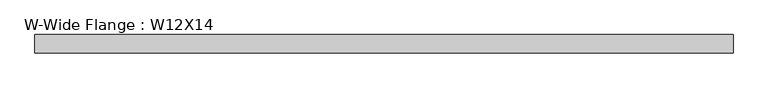
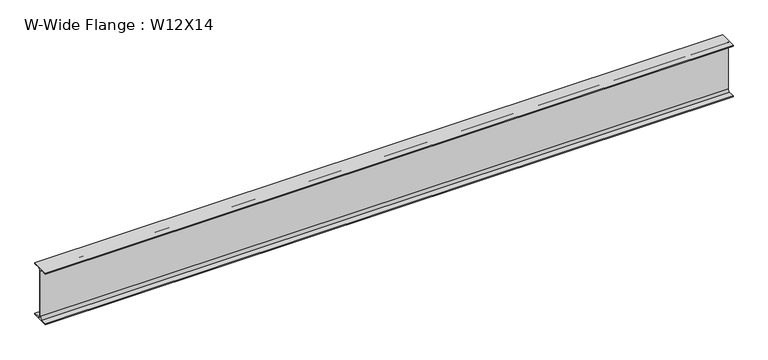
"""IFC4 building model written with IfcOpenShell, lengths in millimetres: beam geometry, W-Wide Flange : W12X14."""

import ifcopenshell
import ifcopenshell.guid

model = None  # the IFC model being written
_history = None  # IfcOwnerHistory: only IFC2X3 demands one
_inside = {}  # id of a spatial element -> (the spatial element, [elements in it])
_under = {}  # id of a project, library or spatial element -> (it, [spatial elements below it])
_declared = {}  # id of a project -> (the project, [libraries it declares])
_typed = {}  # id of a type object -> (the type object, [elements of that type])
_made_of = {}  # id of a material, layer set ... -> (it, [elements and type objects made of it])


def new_model(schema):
    """Start an empty IFC model of exactly this schema.

    Asked for "IFC4X3", IfcOpenShell would pick the latest addendum, in which some entities
    have other attributes; the version numbers below select the first issue.
    IFC2X3 requires an IfcOwnerHistory on every rooted entity: one is made here for all.
    """
    global model, _history
    if schema == "IFC4X3":
        model = ifcopenshell.file(schema_version=(4, 3, 0, 0))
    else:
        model = ifcopenshell.file(schema=schema)
    _inside.clear()
    _under.clear()
    _declared.clear()
    _typed.clear()
    _made_of.clear()
    _history = None
    if model.schema == "IFC2X3":
        org = make("IfcOrganization", Name="unknown")
        user = make(
            "IfcPersonAndOrganization",
            ThePerson=make("IfcPerson", FamilyName="unknown"),
            TheOrganization=org,
        )
        app = make(
            "IfcApplication",
            ApplicationDeveloper=org,
            Version="unknown",
            ApplicationFullName="unknown",
            ApplicationIdentifier="unknown",
        )
        _history = make(
            "IfcOwnerHistory",
            OwningUser=user,
            OwningApplication=app,
            ChangeAction="ADDED",
            CreationDate=0,
        )
    return model


def make(cls, **values):
    """One entity of the class cls with the attributes given. An attribute that is None is left unset."""
    return model.create_entity(
        cls, **{name: value for name, value in values.items() if value is not None}
    )


def rooted(cls, **values):
    """An entity with a GlobalId (a new one), such as an element, a storey or a relation."""
    return make(cls, GlobalId=ifcopenshell.guid.new(), OwnerHistory=_history, **values)


def si_unit(unit_type, name, prefix=None):
    """IfcSIUnit, for example si_unit("LENGTHUNIT", "METRE", prefix="MILLI")."""
    return make("IfcSIUnit", UnitType=unit_type, Prefix=prefix, Name=name)


def assignment(units):
    """IfcUnitAssignment: the units of a project."""
    return None if units is None else make("IfcUnitAssignment", Units=units)


def point(xyz):
    """IfcCartesianPoint."""
    return None if xyz is None else make("IfcCartesianPoint", Coordinates=xyz)


def direction(xyz):
    """IfcDirection."""
    return None if xyz is None else make("IfcDirection", DirectionRatios=xyz)


def frame(location, z_axis=None, x_axis=None):
    """IfcAxis2Placement3D, a coordinate frame: its origin and axes. An axis left out is left unset."""
    return make(
        "IfcAxis2Placement3D",
        Location=point(location),
        Axis=direction(z_axis),
        RefDirection=direction(x_axis),
    )


def frame_2d(location, x_axis=None):
    """IfcAxis2Placement2D, a coordinate frame in the plane: its origin and x axis."""
    return make(
        "IfcAxis2Placement2D", Location=point(location), RefDirection=direction(x_axis)
    )


def origin():
    """The frame at (0, 0, 0) with its axes left unset."""
    return frame((0.0, 0.0, 0.0))


def place(relative_to, where):
    """IfcLocalPlacement: puts the frame where relative to a parent placement (None: the world)."""
    return make(
        "IfcLocalPlacement", PlacementRelTo=relative_to, RelativePlacement=where
    )


def context(
    kind, dimensions, precision=None, world=None, true_north=None, identifier=None
):
    """IfcGeometricRepresentationContext, for example the 3D "Model" context."""
    return make(
        "IfcGeometricRepresentationContext",
        ContextIdentifier=identifier,
        ContextType=kind,
        CoordinateSpaceDimension=dimensions,
        Precision=precision,
        WorldCoordinateSystem=world,
        TrueNorth=true_north,
    )


def project(units=None, contexts=None):
    """IfcProject with its units and contexts."""
    return rooted(
        "IfcProject",
        Name="project",
        RepresentationContexts=contexts,
        UnitsInContext=assignment(units),
    )


def spatial(cls, under=None, at=None, **own):
    """A site, building, storey or space (cls), placed at a placement, below another one or the project."""
    s = rooted(cls, ObjectPlacement=at, **own)
    if under is not None:
        _under.setdefault(under.id(), (under, []))[1].append(s)
    return s


def polyline(points):
    """IfcPolyline through the points."""
    return make("IfcPolyline", Points=[point(p) for p in points])


def circle_curve(where, radius):
    """IfcCircle in the frame where."""
    return make("IfcCircle", Position=where, Radius=radius)


def trimmed(basis, trim1, trim2, sense, master):
    """IfcTrimmedCurve: the piece of a basis curve between two trims."""
    return make(
        "IfcTrimmedCurve",
        BasisCurve=basis,
        Trim1=trim1,
        Trim2=trim2,
        SenseAgreement=sense,
        MasterRepresentation=master,
    )


def segment(curve, same_sense, transition):
    """IfcCompositeCurveSegment."""
    return make(
        "IfcCompositeCurveSegment",
        Transition=transition,
        SameSense=same_sense,
        ParentCurve=curve,
    )


def composite_curve(segments, self_intersect=None):
    """IfcCompositeCurve: segments joined end to end."""
    return make("IfcCompositeCurve", Segments=segments, SelfIntersect=self_intersect)


def outline(outer, holes=None, kind="AREA"):
    """IfcArbitraryClosedProfileDef: a profile drawn as a closed curve; with holes, ...WithVoids."""
    if holes is None:
        return make("IfcArbitraryClosedProfileDef", ProfileType=kind, OuterCurve=outer)
    return make(
        "IfcArbitraryProfileDefWithVoids",
        ProfileType=kind,
        OuterCurve=outer,
        InnerCurves=holes,
    )


def extrude(swept, where, along, depth):
    """IfcExtrudedAreaSolid: the profile swept, set in the frame where, extruded along a direction by depth."""
    return make(
        "IfcExtrudedAreaSolid",
        SweptArea=swept,
        Position=where,
        ExtrudedDirection=direction(along),
        Depth=depth,
    )


def shape(context_of_items, identifier, shape_type, items):
    """IfcShapeRepresentation: the items that make up one representation, for example the "Body"."""
    return make(
        "IfcShapeRepresentation",
        ContextOfItems=context_of_items,
        RepresentationIdentifier=identifier,
        RepresentationType=shape_type,
        Items=items,
    )


def source(mapping_origin, context_of_items, identifier, shape_type, items):
    """IfcRepresentationMap: a shape defined once, which mapped items show again and again."""
    return make(
        "IfcRepresentationMap",
        MappingOrigin=mapping_origin,
        MappedRepresentation=shape(context_of_items, identifier, shape_type, items),
    )


def transform(
    local_origin,
    x_axis=None,
    y_axis=None,
    z_axis=None,
    scale=None,
    scale2=None,
    scale3=None,
    uniform=True,
):
    """IfcCartesianTransformationOperator3D, or its non-uniform kind. x_axis, y_axis, z_axis: its Axis1, 2, 3."""
    if uniform:
        return make(
            "IfcCartesianTransformationOperator3D",
            Axis1=direction(x_axis),
            Axis2=direction(y_axis),
            LocalOrigin=point(local_origin),
            Scale=scale,
            Axis3=direction(z_axis),
        )
    return make(
        "IfcCartesianTransformationOperator3DnonUniform",
        Axis1=direction(x_axis),
        Axis2=direction(y_axis),
        LocalOrigin=point(local_origin),
        Scale=scale,
        Axis3=direction(z_axis),
        Scale2=scale2,
        Scale3=scale3,
    )


def mapped(mapping_source, mapping_target):
    """IfcMappedItem: shows the shape of a source again, moved by a transform."""
    return make(
        "IfcMappedItem", MappingSource=mapping_source, MappingTarget=mapping_target
    )


def made_of(thing, what):
    """Note that an element or type object is made of a material, layer set ...; save() writes the relation."""
    if what is not None:
        _made_of.setdefault(what.id(), (what, []))[1].append(thing)
    return thing


def element(
    cls,
    number,
    at=None,
    inside=None,
    cuts=None,
    type_object=None,
    material=None,
    context=None,
    identifier="Body",
    shape_type=None,
    held_by="IfcProductDefinitionShape",
    body=None,
    shapes=None,
    **own,
):
    """One element of the class cls, such as IfcWall. Its Tag is "e" and its number.

    at: its placement. inside: the storey or other place that contains it. cuts: it is an
    opening in that element (IfcRelVoidsElement). A single representation is given by context,
    identifier, shape_type and body (its items); several are given by shapes. held_by: the class
    of the entity that holds the representations. save() writes the other relations.
    """
    e = rooted(cls, Tag="e%d" % number, ObjectPlacement=at, **own)
    if body is not None:
        shapes = [shape(context, identifier, shape_type, body)]
    if shapes is not None:
        e.Representation = make(held_by, Representations=shapes)
    if inside is not None:
        _inside.setdefault(inside.id(), (inside, []))[1].append(e)
    if cuts is not None:
        rooted(
            "IfcRelVoidsElement", RelatingBuildingElement=cuts, RelatedOpeningElement=e
        )
    if type_object is not None:
        _typed.setdefault(type_object.id(), (type_object, []))[1].append(e)
    return made_of(e, material)


def aggregate(whole, parts):
    """IfcRelAggregates: a whole, such as a stair, and the parts it consists of."""
    return rooted("IfcRelAggregates", RelatingObject=whole, RelatedObjects=parts)


def save(model, path):
    """Write the relations noted so far, then the file.

    IfcRelAggregates (storeys below a building ...), IfcRelContainedInSpatialStructure (elements
    in a storey), IfcRelDefinesByType, IfcRelAssociatesMaterial and IfcRelDeclares: one each for
    every whole, place, type object, material and project.
    """
    for whole, parts in _under.values():
        aggregate(whole, parts)
    for where, things in _inside.values():
        rooted(
            "IfcRelContainedInSpatialStructure",
            RelatedElements=things,
            RelatingStructure=where,
        )
    for kind, things in _typed.values():
        rooted("IfcRelDefinesByType", RelatedObjects=things, RelatingType=kind)
    for what, things in _made_of.values():
        rooted("IfcRelAssociatesMaterial", RelatedObjects=things, RelatingMaterial=what)
    for by, libraries in _declared.values():
        rooted("IfcRelDeclares", RelatingContext=by, RelatedDefinitions=libraries)
    model.write(path)


def w_wide_flange_w12x14_02e3ecd4(model_context):
    return source(origin(), model_context, "Body", "SweptSolid", [
        extrude(outline(composite_curve([segment(polyline([(50.419, -145.415), (50.419, -151.13), (-50.419, -151.13), (-50.419, -145.415), (-15.875, -145.415)]), True, "CONTINUOUS"), segment(trimmed(circle_curve(frame_2d((-15.875, -132.08)), 13.335), [point((-15.875, -145.415))], [point((-2.54, -132.08))], True, "CARTESIAN"), True, "CONTINUOUS"), segment(polyline([(-2.54, -132.08), (-2.54, 132.08)]), True, "CONTINUOUS"), segment(trimmed(circle_curve(frame_2d((-15.875, 132.08)), 13.335), [point((-2.54, 132.08))], [point((-15.875, 145.415))], True, "CARTESIAN"), True, "CONTINUOUS"), segment(polyline([(-15.875, 145.415), (-50.419, 145.415), (-50.419, 151.13), (50.419, 151.13), (50.419, 145.415), (15.875, 145.415)]), True, "CONTINUOUS"), segment(trimmed(circle_curve(frame_2d((15.875, 132.08)), 13.335), [point((15.875, 145.415))], [point((2.54, 132.08))], True, "CARTESIAN"), True, "CONTINUOUS"), segment(polyline([(2.54, 132.08), (2.54, -132.08)]), True, "CONTINUOUS"), segment(trimmed(circle_curve(frame_2d((15.875, -132.08)), 13.335), [point((2.54, -132.08))], [point((15.875, -145.415))], True, "CARTESIAN"), True, "CONTINUOUS"), segment(polyline([(15.875, -145.415), (50.419, -145.415)]), True, "CONTINUOUS")], self_intersect=False)), frame((-1905.0, 0.0, 0.0), z_axis=(1.0, 0.0, 0.0), x_axis=(0.0, 1.0, 0.0)), (0.0, 0.0, 1.0), 3810.0),
    ])


if __name__ == "__main__":
    model = new_model("IFC4")
    model_context = context("Model", 3, world=origin())
    ifc_project = project(units=[si_unit("LENGTHUNIT", "METRE", prefix="MILLI")], contexts=[model_context])
    site = spatial("IfcSite", under=ifc_project)
    building = spatial("IfcBuilding", under=site)
    placement = place(None, origin())
    w_wide_flange_w12x14_shape = w_wide_flange_w12x14_02e3ecd4(model_context)
    element("IfcBeam", 1, ObjectType="W-Wide Flange : W12X14", at=placement, inside=building, context=model_context, shape_type="MappedRepresentation", body=[
        mapped(w_wide_flange_w12x14_shape, transform((0.0, 0.0, 0.0), x_axis=(1.0, 0.0, 0.0), y_axis=(0.0, 1.0, 0.0), z_axis=(0.0, 0.0, 1.0))),
    ])
    save(model, "model.ifc")

# Revit data of these elements
# Type "W-Wide Flange : W12X14"
#   Assembly Code = "B10"
#   W = 14
#   Length [instance default] = 5' - 0"
#   bf = 0' - 3.97"
#   d = 0' - 11.9"
#   k = 0' - 0 3/4"
#   k2 = 0' - 0.525"
#   tf = 0' - 0.225"
#   tw = 0' - 0.2"
#   A = 0.0288889 SF
#   Structural Material [instance default] = Steel ASTM A992
# Element 1 (IfcBeam, "W-Wide Flange : W12X14")
#   Materials on its faces: "Steel ASTM A992"
# Materials
#   "Steel ASTM A992": class "Metal", colour RGB 199 199 199, transparency 0, Description = "Structural steel 50ksi", Cost = 0
